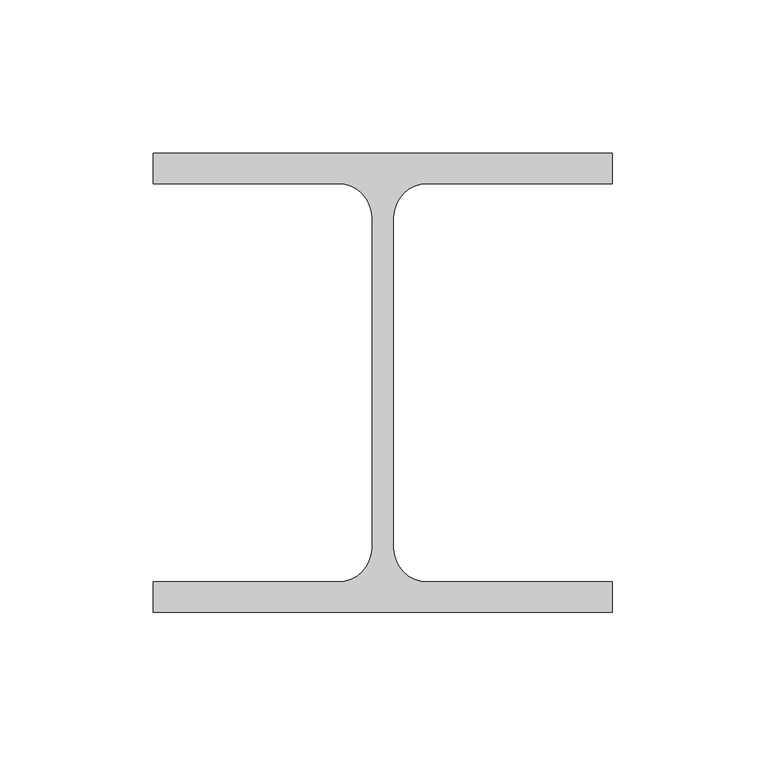
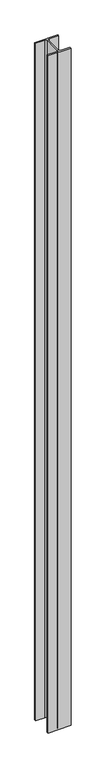
"""IFC4 building model written with IfcOpenShell, lengths in millimetres: column geometry, 0912_Steel Column_H_KSD3502 : H_SC_ASC_H-150x150x7x10."""

from ifc_helpers import new_model, si_unit, point, frame, frame_2d, origin, place, context, project, spatial, polyline, circle_curve, trimmed, segment, composite_curve, outline, extrude, source, transform, mapped, element, save


def column_23aad0d9(model_context):
    return source(origin(), model_context, "Body", "SweptSolid", [
        extrude(outline(composite_curve([segment(polyline([(75.0, 75.0), (75.0, 65.0), (14.5, 65.0)]), True, "CONTINUOUS"), segment(trimmed(circle_curve(frame_2d((14.5, 54.0)), 11.0), [point((14.5, 65.0))], [point((3.5, 54.0))], True, "CARTESIAN"), True, "CONTINUOUS"), segment(polyline([(3.5, 54.0), (3.5, -54.0)]), True, "CONTINUOUS"), segment(trimmed(circle_curve(frame_2d((14.5, -54.0)), 11.0), [point((3.5, -54.0))], [point((14.5, -65.0))], True, "CARTESIAN"), True, "CONTINUOUS"), segment(polyline([(14.5, -65.0), (75.0, -65.0), (75.0, -75.0), (-75.0, -75.0), (-75.0, -65.0), (-14.5, -65.0)]), True, "CONTINUOUS"), segment(trimmed(circle_curve(frame_2d((-14.5, -54.0)), 11.0), [point((-14.5, -65.0))], [point((-3.5, -54.0))], True, "CARTESIAN"), True, "CONTINUOUS"), segment(polyline([(-3.5, -54.0), (-3.5, 54.0)]), True, "CONTINUOUS"), segment(trimmed(circle_curve(frame_2d((-14.5, 54.0)), 11.0), [point((-3.5, 54.0))], [point((-14.5, 65.0))], True, "CARTESIAN"), True, "CONTINUOUS"), segment(polyline([(-14.5, 65.0), (-75.0, 65.0), (-75.0, 75.0), (75.0, 75.0)]), True, "CONTINUOUS")], self_intersect=False)), frame((0.0, 0.0, 12299.9720055), z_axis=(0.0, 0.0, 1.0), x_axis=(1.0, 0.0, 0.0)), (0.0, 0.0, 1.0), 4650.0),
    ])


if __name__ == "__main__":
    model = new_model("IFC4")
    model_context = context("Model", 3, world=origin())
    ifc_project = project(units=[si_unit("LENGTHUNIT", "METRE", prefix="MILLI")], contexts=[model_context])
    site = spatial("IfcSite", under=ifc_project)
    building = spatial("IfcBuilding", under=site)
    placement = place(None, origin())
    column_shape = column_23aad0d9(model_context)
    element("IfcColumn", 1, ObjectType="0912_Steel Column_H_KSD3502 : H_SC_ASC_H-150x150x7x10", at=placement, inside=building, context=model_context, shape_type="MappedRepresentation", body=[
        mapped(column_shape, transform((0.0, 0.0, 0.0), x_axis=(1.0, 0.0, 0.0), y_axis=(0.0, 1.0, 0.0), z_axis=(0.0, 0.0, 1.0))),
    ])
    save(model, "model.ifc")

# Revit data of these elements
# Type "0912_Steel Column_H_KSD3502 : H_SC_ASC_H-150x150x7x10"
#   H_WM Code_1 = "S01AA002-00001 | Main Steel Structure Fabrication Work | Shelter/Building | Medium Steel - Standard (90KG/M>Weight≥30KG/M) | Material: (   )"
#   H_WM Code_2 = "S03AA028-00001 | Main Steel Structure Erection Work | Shelter/Building | Medium Steel (90KG/M>Weight≥30KG/M) | Material: (   )"
#   H_WM Code_3 = "S01AA010-00001 | Main Steel Structure Fabrication Work | Shelter/Building | Steel Painting/Coating | for Non-Fireproofed Steel Surface, Surface Preparation, Primer, Second & Final Coat | Material: (   )"
#   H_Q'ty Cal Type Tag = "SC-Q2"
#   Width = 15.0 cm
#   Web Thickness = 0.7 cm
#   Web Fillet = 1.1 cm
#   Warping Constant = 27562.5 cm⁶
#   Torsional Moment of Inertia = 11.6007 cm⁴
#   Section Area = 40.14 cm²
#   Plastic Modulus weak axis = 115.0 cm³
#   Plastic Modulus strong axis = 246.0 cm³
#   Perimeter = 0.87 m²/m
#   Nominal Weight = 31.50 kgf/m
#   Moment of Inertia weak axis = 563.00 cm⁴
#   Moment of Inertia strong axis = 1640.00 cm⁴
#   Height = 15.0 cm
#   Flange Thickness = 1.0 cm
#   Elastic Modulus weak axis = 75.1 cm³
#   Elastic Modulus strong axis = 219.0 cm³
#   Centroid Vertical = 7.5 cm
#   Centroid Horizontal = 7.5 cm
#   Structural Material [instance default] = Steel, 45-345
#   Section Name Key = ""
#   Bolt Spacing = 0
#   Assembly Code = ""
# Element 1 (IfcColumn, "0912_Steel Column_H_KSD3502 : H_SC_ASC_H-150x150x7x10")
#   Structural Material = none
# Materials
#   "Steel, 45-345": class "Metal", colour RGB 189 187 185, transparency 0, Description = "Steel 345 MPa", Cost = 0
